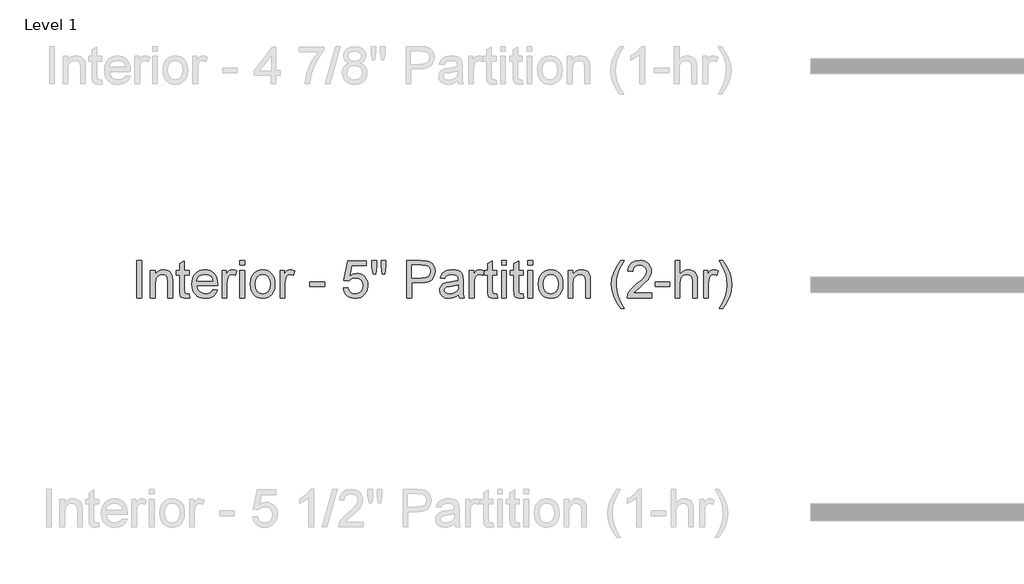
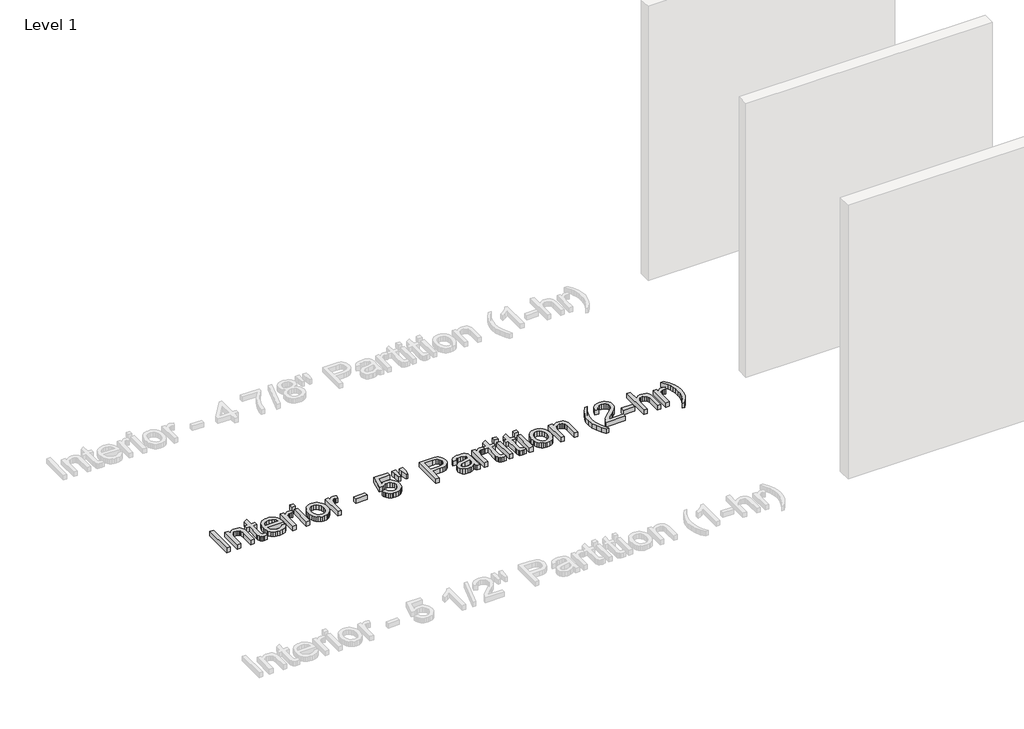
# One storey, part 34 of 42: 1 proxy.
"""IFC4 building model written with IfcOpenShell, lengths in millimetres."""

from ifc_helpers import new_model, si_unit, origin, origin_with_axes, place, context, project, spatial, polyline, outline, extrude, element, save

model = new_model("IFC4")

# Units and contexts
model_context = context("Model", 3, world=origin())
ifc_project = project(units=[si_unit("LENGTHUNIT", "METRE", prefix="MILLI")], contexts=[model_context])

# Site, building, storey
site = spatial("IfcSite", under=ifc_project)
building = spatial("IfcBuilding", under=site)
storey = spatial("IfcBuildingStorey", under=building, Name="Level 1", Elevation=0.0)

# Proxy
placement = place(None, origin())
element("IfcBuildingElementProxy", 1, Name="8\" Arial", ObjectType="8\" Arial", at=placement, inside=storey, context=model_context, shape_type="SweptSolid", body=[
    extrude(outline(polyline([(6003.2577476, 11994.6253326), (6003.2577476, 12299.1924266), (6041.3286344, 12299.1924266), (6041.3286344, 11994.6253326), (6003.2577476, 11994.6253326)])), origin_with_axes(), (0.0, 0.0, 1.0), 50.8),
    extrude(outline(polyline([(6112.711547, 11994.6253326), (6112.711547, 12218.2917923), (6150.7824338, 12218.2917923), (6150.7824338, 12187.061768), (6164.0087209, 12202.8069052), (6179.8932779, 12214.0534318), (6198.4361048, 12220.8013478), (6219.6372016, 12223.0506531), (6238.4031002, 12221.2381963), (6255.5889082, 12215.800826), (6269.9212586, 12207.4170517), (6280.1267844, 12196.7653827), (6291.5406147, 12168.7698966), (6293.5482591, 12131.9630822), (6293.5482591, 11994.6253326), (6255.4773724, 11994.6253326), (6255.4773724, 12126.8324354), (6251.0902975, 12160.5162473), (6245.020891, 12170.5451748), (6235.5868212, 12178.3247969), (6223.4944814, 12183.316024), (6209.4502651, 12184.9797663), (6187.1523996, 12181.243317), (6168.1448402, 12170.033969), (6160.5487874, 12160.883386), (6155.1230354, 12148.3774343), (6150.7824338, 12113.2994249), (6150.7824338, 11994.6253326), (6112.711547, 11994.6253326)])), origin_with_axes(), (0.0, 0.0, 1.0), 50.8),
    extrude(outline(polyline([(6426.7963628, 12026.3758573), (6431.5552236, 11993.5099745), (6403.0764158, 11989.8664717), (6384.8031337, 11991.4465622), (6371.1771767, 11996.1868338), (6361.5479192, 12003.4924287), (6355.2647357, 12012.7684895), (6351.8071259, 12028.6995198), (6350.6545893, 12055.9700231), (6350.6545893, 12180.2209055), (6322.1014242, 12180.2209055), (6322.1014242, 12218.2917923), (6350.6545893, 12218.2917923), (6350.6545893, 12272.646906), (6388.725476, 12295.0284234), (6388.725476, 12218.2917923), (6426.7963628, 12218.2917923), (6426.7963628, 12180.2209055), (6388.725476, 12180.2209055), (6388.725476, 12057.0853811), (6390.7331204, 12037.4550802), (6397.2393755, 12030.5026819), (6410.214707, 12027.9373585), (6426.7963628, 12026.3758573)])), origin_with_axes(), (0.0, 0.0, 1.0), 50.8),
    extrude(outline(polyline([(6621.4635142, 12061.2493844), (6658.790829, 12056.4905235), (6645.3414703, 12028.3649124), (6623.8801232, 12007.3404139), (6594.8901096, 11994.2349572), (6558.8547512, 11989.8664717), (6535.232398, 11991.750962), (6514.1846629, 11997.4044329), (6495.7115459, 12006.8268845), (6479.8130469, 12020.0183166), (6467.0282557, 12036.6115907), (6457.896262, 12056.239568), (6452.4170658, 12078.9022486), (6450.590667, 12104.5996324), (6452.4356551, 12131.1683897), (6457.9706192, 12154.5862606), (6467.1955594, 12174.8532451), (6480.1104757, 12191.9693432), (6495.9671487, 12205.5674163), (6514.0173592, 12215.2803256), (6534.2611071, 12221.1080712), (6556.6983924, 12223.0506531), (6578.4130187, 12221.1127186), (6598.0502907, 12215.2989149), (6615.6102083, 12205.6092422), (6631.0927717, 12192.0437004), (6643.7311722, 12174.9647809), (6652.7586011, 12154.734975), (6658.1750584, 12131.3542827), (6659.9805442, 12104.822704), (6659.7574726, 12094.5614103), (6488.6615538, 12094.5614103), (6495.2514607, 12066.0640131), (6510.5597494, 12045.1138718), (6532.6531326, 12032.2314868), (6559.5983232, 12027.9373585), (6579.8606604, 12029.9264136), (6596.925638, 12035.8935789), (6610.7932559, 12046.2106405), (6621.4635142, 12061.2493844)]), holes=[polyline([(6488.6615538, 12132.6322971), (6621.9096574, 12132.6322971), (6616.7604213, 12152.7459198), (6606.6664313, 12167.1340382), (6584.4708069, 12180.5183343), (6556.549678, 12184.9797663), (6530.8871491, 12181.4199154), (6509.667463, 12170.7403624), (6494.9168533, 12154.0936441), (6488.6615538, 12132.6322971)])]), origin_with_axes(), (0.0, 0.0, 1.0), 50.8),
    extrude(outline(polyline([(6698.0514309, 11994.6253326), (6698.0514309, 12218.2917923), (6731.3634569, 12218.2917923), (6731.3634569, 12185.2028379), (6743.6695736, 12204.3869957), (6755.0090467, 12215.6892902), (6766.3856984, 12221.2103124), (6778.8033509, 12223.0506531), (6797.7644371, 12220.1135437), (6817.0229521, 12211.3022154), (6804.3078707, 12177.1722603), (6790.9235746, 12183.0278898), (6777.5392785, 12184.9797663), (6766.1719214, 12183.102247), (6756.0128689, 12177.4696891), (6747.8056929, 12168.5096464), (6742.2939654, 12156.6496729), (6737.6652296, 12135.3835135), (6736.1223177, 12112.1840669), (6736.1223177, 11994.6253326), (6698.0514309, 11994.6253326)])), origin_with_axes(), (0.0, 0.0, 1.0), 50.8),
    extrude(outline(polyline([(6840.8172563, 12261.1215399), (6840.8172563, 12299.1924266), (6878.888143, 12299.1924266), (6878.888143, 12261.1215399), (6840.8172563, 12261.1215399)])), origin_with_axes(), (0.0, 0.0, 1.0), 50.8),
    extrude(outline(polyline([(6840.8172563, 11994.6253326), (6840.8172563, 12218.2917923), (6878.888143, 12218.2917923), (6878.888143, 11994.6253326), (6840.8172563, 11994.6253326)])), origin_with_axes(), (0.0, 0.0, 1.0), 50.8),
    extrude(outline(polyline([(6926.4767515, 12106.4585624), (6928.5355165, 12135.4253394), (6934.7118115, 12160.3861222), (6945.0056364, 12181.3409108), (6959.4169914, 12198.2897053), (6973.9259402, 12209.1226199), (6989.9406223, 12216.8604161), (7007.4610377, 12221.5030939), (7026.4871864, 12223.0506531), (7047.490772, 12221.1661628), (7066.4820658, 12215.5126919), (7083.4610678, 12206.0902404), (7098.4277781, 12192.8988082), (7110.643272, 12176.3845387), (7119.3686248, 12156.9935749), (7124.6038364, 12134.725917), (7126.348907, 12109.5815648), (7123.2630831, 12071.1203028), (7114.0056117, 12041.842155), (7098.8460374, 12019.9160754), (7078.0539051, 12003.511018), (7053.3580198, 11993.2776083), (7026.4871864, 11989.8664717), (7005.1768774, 11991.743991), (6986.0089853, 11997.376549), (6968.98351, 12006.7641456), (6954.1004516, 12019.9067808), (6942.0150828, 12036.581383), (6933.3826765, 12056.5648807), (6928.2032327, 12079.8572739), (6926.4767515, 12106.4585624)]), holes=[polyline([(6964.5476383, 12106.5329196), (6968.9533024, 12072.0776517), (6982.1702948, 12047.5304809), (7002.060846, 12032.8356391), (7026.4871864, 12027.9373585), (7050.8019911, 12032.863523), (7070.6553637, 12047.6420167), (7083.8723561, 12072.5145003), (7088.2780202, 12107.7226348), (7083.8444721, 12141.1740805), (7070.5438279, 12165.386644), (7050.6625713, 12180.0814857), (7026.4871864, 12184.9797663), (7002.060846, 12180.100075), (6982.1702948, 12165.4610012), (6968.9533024, 12140.9695982), (6964.5476383, 12106.5329196)])]), origin_with_axes(), (0.0, 0.0, 1.0), 50.8),
    extrude(outline(polyline([(7169.1786546, 11994.6253326), (7169.1786546, 12218.2917923), (7202.4906805, 12218.2917923), (7202.4906805, 12185.2028379), (7214.7967972, 12204.3869957), (7226.1362703, 12215.6892902), (7237.512922, 12221.2103124), (7249.9305745, 12223.0506531), (7268.8916607, 12220.1135437), (7288.1501757, 12211.3022154), (7275.4350944, 12177.1722603), (7262.0507983, 12183.0278898), (7248.6665021, 12184.9797663), (7237.2991451, 12183.102247), (7227.1400925, 12177.4696891), (7218.9329165, 12168.5096464), (7213.421189, 12156.6496729), (7208.7924533, 12135.3835135), (7207.2495413, 12112.1840669), (7207.2495413, 11994.6253326), (7169.1786546, 11994.6253326)])), origin_with_axes(), (0.0, 0.0, 1.0), 50.8),
    extrude(outline(polyline([(7411.8805577, 12085.0436886), (7411.8805577, 12123.1145754), (7530.8520788, 12123.1145754), (7530.8520788, 12085.0436886), (7411.8805577, 12085.0436886)])), origin_with_axes(), (0.0, 0.0, 1.0), 50.8),
    extrude(outline(polyline([(7683.1356258, 12075.5259669), (7721.2065126, 12080.2848278), (7728.1960894, 12057.4292832), (7740.3906704, 12041.0614044), (7757.7344874, 12031.2183699), (7780.1717727, 12027.9373585), (7807.4608654, 12032.5010317), (7827.9090956, 12046.1920512), (7840.6799448, 12067.4303267), (7844.9368945, 12094.6357675), (7840.9494897, 12120.2518231), (7828.987275, 12139.8449455), (7808.9573041, 12152.2811873), (7780.7666303, 12156.4266013), (7762.2981606, 12154.7721536), (7747.3430686, 12149.8088104), (7725.9653734, 12132.6322971), (7687.8944867, 12137.3911579), (7721.2065126, 12294.4335658), (7868.7311988, 12294.4335658), (7868.7311988, 12256.362679), (7751.9903937, 12256.362679), (7735.7061667, 12172.4877566), (7762.9023129, 12188.9950552), (7791.39971, 12194.497488), (7809.9402133, 12192.7919197), (7826.9703359, 12187.6752149), (7842.4900779, 12179.1473734), (7856.4994393, 12167.2083954), (7868.0968389, 12152.5879108), (7876.3806958, 12136.0155497), (7881.3510099, 12117.4913121), (7883.0077813, 12097.0151979), (7877.0406159, 12058.9443112), (7869.5816593, 12041.9722801), (7859.1391199, 12026.3758573), (7843.3196254, 12010.4030011), (7824.8604504, 11998.9938181), (7803.7615947, 11992.1483083), (7780.0230583, 11989.8664717), (7760.3764917, 11991.3327028), (7742.630681, 11995.7313959), (7726.7856263, 12003.0625512), (7712.8413275, 12013.3261685), (7701.2392805, 12026.0110422), (7692.4209813, 12040.6059665), (7686.3864297, 12057.1109414), (7683.1356258, 12075.5259669)])), origin_with_axes(), (0.0, 0.0, 1.0), 50.8),
    extrude(outline(polyline([(7925.6144573, 12189.7386272), (7916.3198072, 12248.5551729), (7916.3198072, 12299.1924266), (7954.390694, 12299.1924266), (7954.390694, 12248.5551729), (7946.0626875, 12189.7386272), (7925.6144573, 12189.7386272)])), origin_with_axes(), (0.0, 0.0, 1.0), 50.8),
    extrude(outline(polyline([(8001.5331592, 12189.7386272), (7992.4615807, 12248.5551729), (7992.4615807, 12299.1924266), (8030.5324675, 12299.1924266), (8030.5324675, 12248.5551729), (8021.6096034, 12189.7386272), (8001.5331592, 12189.7386272)])), origin_with_axes(), (0.0, 0.0, 1.0), 50.8),
    extrude(outline(polyline([(8201.8514579, 11994.6253326), (8201.8514579, 12299.1924266), (8314.7256886, 12299.1924266), (8360.2322954, 12296.2924958), (8380.5225165, 12290.8737148), (8397.2250027, 12282.0530919), (8410.6743614, 12269.430957), (8421.2052, 12252.6076404), (8428.0088838, 12232.7635624), (8430.2767785, 12211.0791438), (8428.7454849, 12192.3829551), (8424.151604, 12175.1832052), (8416.495136, 12159.4798938), (8405.7760808, 12145.2730212), (8391.0603261, 12133.4966995), (8371.4137595, 12125.0850412), (8346.836381, 12120.0380462), (8317.3281906, 12118.3557145), (8239.9223447, 12118.3557145), (8239.9223447, 11994.6253326), (8201.8514579, 11994.6253326)]), holes=[polyline([(8239.9223447, 12156.4266013), (8319.5589066, 12156.4266013), (8353.3170757, 12159.9213897), (8375.6242359, 12170.405755), (8388.0604778, 12187.2290717), (8392.2058917, 12209.7407142), (8389.7613987, 12226.8428703), (8382.4279198, 12241.2681673), (8371.1163306, 12252.1243186), (8356.737507, 12258.5190378), (8318.6666202, 12261.1215399), (8239.9223447, 12261.1215399), (8239.9223447, 12156.4266013)])]), origin_with_axes(), (0.0, 0.0, 1.0), 50.8),
    extrude(outline(polyline([(8620.6312122, 12023.1784976), (8602.441582, 12007.5820748), (8583.7128621, 11997.376549), (8564.0174986, 11991.743991), (8542.9279375, 11989.8664717), (8511.1123503, 11994.3836716), (8487.6433588, 12007.9352715), (8473.1715886, 12028.5136268), (8468.3476652, 12054.1110931), (8470.1694166, 12069.893409), (8475.6346709, 12084.2257594), (8484.0649185, 12096.4946975), (8494.7816501, 12106.0867764), (8521.4387065, 12118.5787861), (8554.3789464, 12124.3042906), (8593.304941, 12130.3272238), (8620.4081406, 12137.3911579), (8620.6312122, 12145.8678788), (8618.0101209, 12162.8584991), (8610.146847, 12173.9749006), (8592.561369, 12182.2285499), (8568.0606714, 12184.9797663), (8545.3817251, 12183.1487203), (8529.5436414, 12177.6555821), (8518.743258, 12167.4965295), (8511.1774128, 12151.6677404), (8473.1065261, 12156.4266013), (8479.7150223, 12177.2466175), (8489.576646, 12193.6052016), (8503.6115676, 12206.1158006), (8522.7399575, 12215.3918614), (8546.1345918, 12221.1359552), (8572.9682466, 12223.0506531), (8598.7051327, 12221.3590268), (8619.1068896, 12216.2841478), (8634.4895355, 12208.6532401), (8645.1690885, 12199.2935275), (8652.2516118, 12187.7216881), (8656.843169, 12173.4544002), (8658.702099, 12140.1423743), (8658.702099, 12092.7768375), (8660.6353862, 12026.6361075), (8668.2198207, 11994.6253326), (8630.1489339, 11994.6253326), (8624.0516435, 12007.8609143), (8620.6312122, 12023.1784976)]), holes=[polyline([(8620.6312122, 12099.3202711), (8559.2121645, 12087.6461906), (8526.4578176, 12081.474543), (8511.623556, 12071.4363209), (8506.418552, 12056.7879523), (8509.2534202, 12045.4670685), (8517.7580251, 12036.1910077), (8531.7464735, 12030.0007708), (8551.0328724, 12027.9373585), (8571.4811026, 12030.2145477), (8589.5499024, 12037.0461156), (8604.1982709, 12047.1122216), (8614.3852074, 12059.0930256), (8618.9024073, 12071.4363209), (8620.4081406, 12088.538477), (8620.6312122, 12099.3202711)])]), origin_with_axes(), (0.0, 0.0, 1.0), 50.8),
    extrude(outline(polyline([(8711.0495683, 11994.6253326), (8711.0495683, 12218.2917923), (8744.3615942, 12218.2917923), (8744.3615942, 12185.2028379), (8756.6677109, 12204.3869957), (8768.007184, 12215.6892902), (8779.3838357, 12221.2103124), (8791.8014883, 12223.0506531), (8810.7625744, 12220.1135437), (8830.0210894, 12211.3022154), (8817.3060081, 12177.1722603), (8803.921712, 12183.0278898), (8790.5374158, 12184.9797663), (8779.1700588, 12183.102247), (8769.0110062, 12177.4696891), (8760.8038302, 12168.5096464), (8755.2921027, 12156.6496729), (8750.663367, 12135.3835135), (8749.1204551, 12112.1840669), (8749.1204551, 11994.6253326), (8711.0495683, 11994.6253326)])), origin_with_axes(), (0.0, 0.0, 1.0), 50.8),
    extrude(outline(polyline([(8934.716028, 12026.3758573), (8939.4748889, 11993.5099745), (8910.996081, 11989.8664717), (8892.7227989, 11991.4465622), (8879.0968419, 11996.1868338), (8869.4675844, 12003.4924287), (8863.1844009, 12012.7684895), (8859.7267911, 12028.6995198), (8858.5742545, 12055.9700231), (8858.5742545, 12180.2209055), (8830.0210894, 12180.2209055), (8830.0210894, 12218.2917923), (8858.5742545, 12218.2917923), (8858.5742545, 12272.646906), (8896.6451412, 12295.0284234), (8896.6451412, 12218.2917923), (8934.716028, 12218.2917923), (8934.716028, 12180.2209055), (8896.6451412, 12180.2209055), (8896.6451412, 12057.0853811), (8898.6527857, 12037.4550802), (8905.1590407, 12030.5026819), (8918.1343723, 12027.9373585), (8934.716028, 12026.3758573)])), origin_with_axes(), (0.0, 0.0, 1.0), 50.8),
    extrude(outline(polyline([(8972.7869148, 11994.6253326), (8972.7869148, 12218.2917923), (9010.8578015, 12218.2917923), (9010.8578015, 11994.6253326), (8972.7869148, 11994.6253326)])), origin_with_axes(), (0.0, 0.0, 1.0), 50.8),
    extrude(outline(polyline([(8972.7869148, 12261.1215399), (8972.7869148, 12299.1924266), (9010.8578015, 12299.1924266), (9010.8578015, 12261.1215399), (8972.7869148, 12261.1215399)])), origin_with_axes(), (0.0, 0.0, 1.0), 50.8),
    extrude(outline(polyline([(9148.864766, 12026.3758573), (9153.6236269, 11993.5099745), (9125.144819, 11989.8664717), (9106.8715369, 11991.4465622), (9093.2455799, 11996.1868338), (9083.6163224, 12003.4924287), (9077.3331389, 12012.7684895), (9073.8755291, 12028.6995198), (9072.7229925, 12055.9700231), (9072.7229925, 12180.2209055), (9044.1698274, 12180.2209055), (9044.1698274, 12218.2917923), (9072.7229925, 12218.2917923), (9072.7229925, 12272.646906), (9110.7938793, 12295.0284234), (9110.7938793, 12218.2917923), (9148.864766, 12218.2917923), (9148.864766, 12180.2209055), (9110.7938793, 12180.2209055), (9110.7938793, 12057.0853811), (9112.8015237, 12037.4550802), (9119.3077787, 12030.5026819), (9132.2831103, 12027.9373585), (9148.864766, 12026.3758573)])), origin_with_axes(), (0.0, 0.0, 1.0), 50.8),
    extrude(outline(polyline([(9186.9356528, 12261.1215399), (9186.9356528, 12299.1924266), (9225.0065395, 12299.1924266), (9225.0065395, 12261.1215399), (9186.9356528, 12261.1215399)])), origin_with_axes(), (0.0, 0.0, 1.0), 50.8),
    extrude(outline(polyline([(9186.9356528, 11994.6253326), (9186.9356528, 12218.2917923), (9225.0065395, 12218.2917923), (9225.0065395, 11994.6253326), (9186.9356528, 11994.6253326)])), origin_with_axes(), (0.0, 0.0, 1.0), 50.8),
    extrude(outline(polyline([(9272.595148, 12106.4585624), (9274.653913, 12135.4253394), (9280.830208, 12160.3861222), (9291.1240329, 12181.3409108), (9305.5353879, 12198.2897053), (9320.0443367, 12209.1226199), (9336.0590188, 12216.8604161), (9353.5794342, 12221.5030939), (9372.6055829, 12223.0506531), (9393.6091685, 12221.1661628), (9412.6004623, 12215.5126919), (9429.5794643, 12206.0902404), (9444.5461746, 12192.8988082), (9456.7616685, 12176.3845387), (9465.4870213, 12156.9935749), (9470.7222329, 12134.725917), (9472.4673035, 12109.5815648), (9469.3814796, 12071.1203028), (9460.1240082, 12041.842155), (9444.9644339, 12019.9160754), (9424.1723016, 12003.511018), (9399.4764163, 11993.2776083), (9372.6055829, 11989.8664717), (9351.2952739, 11991.743991), (9332.1273818, 11997.376549), (9315.1019065, 12006.7641456), (9300.218848, 12019.9067808), (9288.1334793, 12036.581383), (9279.501073, 12056.5648807), (9274.3216292, 12079.8572739), (9272.595148, 12106.4585624)]), holes=[polyline([(9310.6660347, 12106.5329196), (9315.0716989, 12072.0776517), (9328.2886913, 12047.5304809), (9348.1792425, 12032.8356391), (9372.6055829, 12027.9373585), (9396.9203876, 12032.863523), (9416.7737601, 12047.6420167), (9429.9907526, 12072.5145003), (9434.3964167, 12107.7226348), (9429.9628686, 12141.1740805), (9416.6622243, 12165.386644), (9396.7809678, 12180.0814857), (9372.6055829, 12184.9797663), (9348.1792425, 12180.100075), (9328.2886913, 12165.4610012), (9315.0716989, 12140.9695982), (9310.6660347, 12106.5329196)])]), origin_with_axes(), (0.0, 0.0, 1.0), 50.8),
    extrude(outline(polyline([(9515.2970511, 11994.6253326), (9515.2970511, 12218.2917923), (9553.3679378, 12218.2917923), (9553.3679378, 12187.061768), (9566.5942249, 12202.8069052), (9582.4787819, 12214.0534318), (9601.0216088, 12220.8013478), (9622.2227057, 12223.0506531), (9640.9886042, 12221.2381963), (9658.1744122, 12215.800826), (9672.5067627, 12207.4170517), (9682.7122885, 12196.7653827), (9694.1261188, 12168.7698966), (9696.1337632, 12131.9630822), (9696.1337632, 11994.6253326), (9658.0628764, 11994.6253326), (9658.0628764, 12126.8324354), (9653.6758016, 12160.5162473), (9647.6063951, 12170.5451748), (9638.1723252, 12178.3247969), (9626.0799855, 12183.316024), (9612.0357692, 12184.9797663), (9589.7379036, 12181.243317), (9570.7303442, 12170.033969), (9563.1342914, 12160.883386), (9557.7085394, 12148.3774343), (9553.3679378, 12113.2994249), (9553.3679378, 11994.6253326), (9515.2970511, 11994.6253326)])), origin_with_axes(), (0.0, 0.0, 1.0), 50.8),
    extrude(outline(polyline([(9943.5945271, 11908.9658373), (9914.0933077, 11950.3642088), (9889.5368422, 11998.2688354), (9872.9737757, 12050.3560545), (9867.4527536, 12104.3022036), (9871.5795782, 12151.6119725), (9883.9600521, 12196.8769185), (9908.535107, 12248.1462083), (9943.5945271, 12299.1924266), (9972.1476922, 12299.1924266), (9936.530593, 12238.8887369), (9915.1157192, 12180.4439771), (9907.9216601, 12142.354501), (9905.5236403, 12104.079132), (9909.6876436, 12055.2729244), (9922.1796533, 12006.4853061), (9942.9996695, 11957.7162771), (9972.1476922, 11908.9658373), (9943.5945271, 11908.9658373)])), origin_with_axes(), (0.0, 0.0, 1.0), 50.8),
    extrude(outline(polyline([(10195.8141519, 12032.6962193), (10195.8141519, 11994.6253326), (9995.9419964, 11994.6253326), (10000.0316424, 12020.8734244), (10009.419239, 12041.3867171), (10023.1567319, 12061.286563), (10043.0286937, 12082.1158738), (10070.8196975, 12105.4175616), (10111.9020509, 12141.9083578), (10136.5514629, 12168.8442538), (10148.8761689, 12190.7052708), (10152.9844043, 12211.9714302), (10149.1085352, 12231.0347575), (10137.4809279, 12246.8821359), (10119.6073158, 12257.5616889), (10096.9934322, 12261.1215399), (10073.2456012, 12257.6453407), (10054.7957208, 12247.2167433), (10042.889274, 12230.6536769), (10038.771744, 12208.7740706), (10000.7008572, 12213.5329314), (10003.9748977, 12233.186469), (10009.9304448, 12250.3583351), (10018.5674984, 12265.0485295), (10029.8860585, 12277.2570524), (10043.625875, 12286.8537786), (10059.5266976, 12293.7085831), (10097.8113614, 12299.1924266), (10118.215442, 12297.668104), (10136.3748646, 12293.0951362), (10152.2896292, 12285.4735231), (10165.9597358, 12274.8032648), (10176.9390412, 12261.8744065), (10184.7814022, 12247.4769935), (10189.4868188, 12231.6110258), (10191.055291, 12214.2765034), (10189.3636647, 12196.0682839), (10184.2887858, 12178.1760825), (10175.2822698, 12159.9771576), (10161.7957326, 12140.8487677), (10140.2972069, 12118.0118125), (10107.2547258, 12088.6871914), (10063.4583346, 12052.0662701), (10046.2818213, 12032.6962193), (10195.8141519, 12032.6962193)])), origin_with_axes(), (0.0, 0.0, 1.0), 50.8),
    extrude(outline(polyline([(10224.367317, 12085.0436886), (10224.367317, 12123.1145754), (10343.3388381, 12123.1145754), (10343.3388381, 12085.0436886), (10224.367317, 12085.0436886)])), origin_with_axes(), (0.0, 0.0, 1.0), 50.8),
    extrude(outline(polyline([(10386.1685857, 11994.6253326), (10386.1685857, 12299.1924266), (10424.2394724, 12299.1924266), (10424.2394724, 12187.2104824), (10438.2232735, 12202.8905571), (10453.9265848, 12214.0906104), (10471.3494064, 12220.8106424), (10490.4917383, 12223.0506531), (10513.4867026, 12220.6061601), (10533.2471287, 12213.2726812), (10548.8063729, 12201.6264847), (10559.1977917, 12186.2438388), (10565.0534213, 12165.1078045), (10567.0052978, 12136.2014427), (10567.0052978, 11994.6253326), (10528.934411, 11994.6253326), (10528.934411, 12132.260511), (10525.9043551, 12156.0919939), (10516.8141873, 12172.4133994), (10502.1658188, 12181.8381746), (10482.4611606, 12184.9797663), (10466.3721213, 12182.8605861), (10451.2683149, 12176.5030455), (10438.7577159, 12166.5205913), (10430.4482987, 12153.5266704), (10425.791679, 12136.2572106), (10424.2394724, 12113.4481393), (10424.2394724, 11994.6253326), (10386.1685857, 11994.6253326)])), origin_with_axes(), (0.0, 0.0, 1.0), 50.8),
    extrude(outline(polyline([(10619.3527671, 11994.6253326), (10619.3527671, 12218.2917923), (10652.664793, 12218.2917923), (10652.664793, 12185.2028379), (10664.9709097, 12204.3869957), (10676.3103828, 12215.6892902), (10687.6870345, 12221.2103124), (10700.104687, 12223.0506531), (10719.0657732, 12220.1135437), (10738.3242882, 12211.3022154), (10725.6092069, 12177.1722603), (10712.2249107, 12183.0278898), (10698.8406146, 12184.9797663), (10687.4732576, 12183.102247), (10677.314205, 12177.4696891), (10669.107029, 12168.5096464), (10663.5953015, 12156.6496729), (10658.9665657, 12135.3835135), (10657.4236538, 12112.1840669), (10657.4236538, 11994.6253326), (10619.3527671, 11994.6253326)])), origin_with_axes(), (0.0, 0.0, 1.0), 50.8),
    extrude(outline(polyline([(10771.6363141, 11908.9658373), (10743.083149, 11908.9658373), (10772.2311717, 11957.7162771), (10793.0511879, 12006.4853061), (10805.5431976, 12055.2729244), (10809.7072009, 12104.079132), (10807.3091811, 12142.0756615), (10800.115122, 12179.7747623), (10791.0249542, 12209.6477677), (10778.9233198, 12238.2938792), (10743.083149, 12299.1924266), (10771.6363141, 12299.1924266), (10806.6957342, 12248.1462083), (10831.2707891, 12196.8769185), (10843.651263, 12151.6119725), (10847.7780876, 12104.3022036), (10842.2291815, 12050.3560545), (10825.5824632, 11998.2688354), (10800.9981137, 11950.3642088), (10771.6363141, 11908.9658373)])), origin_with_axes(), (0.0, 0.0, 1.0), 50.8),
])

save(model, "model.ifc")

# Revit data of these elements
# Element 1 (IfcBuildingElementProxy, "8\" Arial")
#   Phase Created = New Construction
